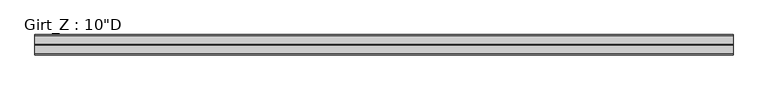
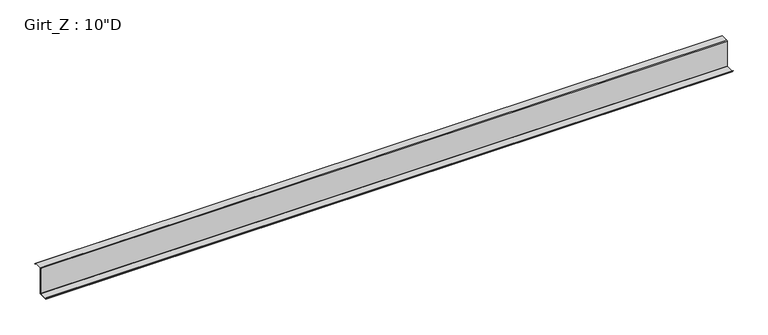
"""IFC4 building model written with IfcOpenShell, lengths in millimetres: beam geometry."""

from ifc_helpers import new_model, si_unit, point, frame, frame_2d, origin, place, context, project, spatial, polyline, circle_curve, trimmed, segment, composite_curve, outline, extrude, source, transform, mapped, element, save


def beam_42cbf969(model_context):
    return source(origin(), model_context, "Body", "SweptSolid", [
        extrude(outline(composite_curve([segment(polyline([(77.9859375, 127.0), (90.2310415, 112.4068534), (88.1028742, 110.621109), (76.6904765, 124.221875), (3.3005807, 124.221875)]), True, "CONTINUOUS"), segment(trimmed(circle_curve(frame_2d((3.3741066, 122.2381931)), 1.9850441), [point((3.3005807, 124.221875))], [point((1.3890625, 122.2381931))], True, "CARTESIAN"), True, "CONTINUOUS"), segment(polyline([(1.3890625, 122.2381931), (1.3890625, -127.0), (-84.3359375, -127.0), (-96.5810415, -112.4068534), (-94.4528742, -110.621109), (-83.0404765, -124.221875), (-3.2694106, -124.221875)]), True, "CONTINUOUS"), segment(trimmed(circle_curve(frame_2d((-3.3748024, -122.2389339)), 1.9857399), [point((-3.2694106, -124.221875))], [point((-1.3890625, -122.2389339))], True, "CARTESIAN"), True, "CONTINUOUS"), segment(polyline([(-1.3890625, -122.2389339), (-1.3890625, 122.2375)]), True, "CONTINUOUS"), segment(trimmed(circle_curve(frame_2d((3.3734375, 122.2375)), 4.7625), [point((-1.3890625, 122.2375))], [point((3.3734375, 127.0))], False, "CARTESIAN"), True, "CONTINUOUS"), segment(polyline([(3.3734375, 127.0), (77.9859375, 127.0)]), True, "CONTINUOUS")], self_intersect=False)), frame((-3200.4, 0.0, 0.0), z_axis=(1.0, 0.0, 0.0), x_axis=(0.0, 1.0, 0.0)), (0.0, 0.0, 1.0), 6356.35),
    ])


if __name__ == "__main__":
    model = new_model("IFC4")
    model_context = context("Model", 3, world=origin())
    ifc_project = project(units=[si_unit("LENGTHUNIT", "METRE", prefix="MILLI")], contexts=[model_context])
    site = spatial("IfcSite", under=ifc_project)
    building = spatial("IfcBuilding", under=site)
    placement = place(None, origin())
    beam_shape = beam_42cbf969(model_context)
    element("IfcBeam", 1, ObjectType="Girt_Z : 10\"D", at=placement, inside=building, context=model_context, shape_type="MappedRepresentation", body=[
        mapped(beam_shape, transform((0.0, 0.0, 0.0), x_axis=(1.0, 0.0, 0.0), y_axis=(0.0, 1.0, 0.0), z_axis=(0.0, 0.0, 1.0))),
    ])
    save(model, "model.ifc")

# Revit data of these elements
# Type "Girt_Z : 10\"D"
#   half leg = 0' - 1 11/16"
#   Web_Thickness = 0' - 0 7/64"
#   Length [instance default] = 10' - 0"
#   Leg_2 = 0' - 3 3/8"
#   Leg_1 = 0' - 3 1/8"
#   Height = 0' - 10"
#   Structural Material [instance default] = none
# Element 1 (IfcBeam, "Girt_Z : 10\"D")
#   Structural Material = STRUCTURAL STEEL - SEE STRUCT. DWGS
#   Materials on its faces: "STRUCTURAL STEEL - SEE STRUCT. DWGS"
# Materials
#   "STRUCTURAL STEEL - SEE STRUCT. DWGS": class "Metal", colour RGB 137 146 153, transparency 0, Description = "Steel, mill finish", Cost = 0
